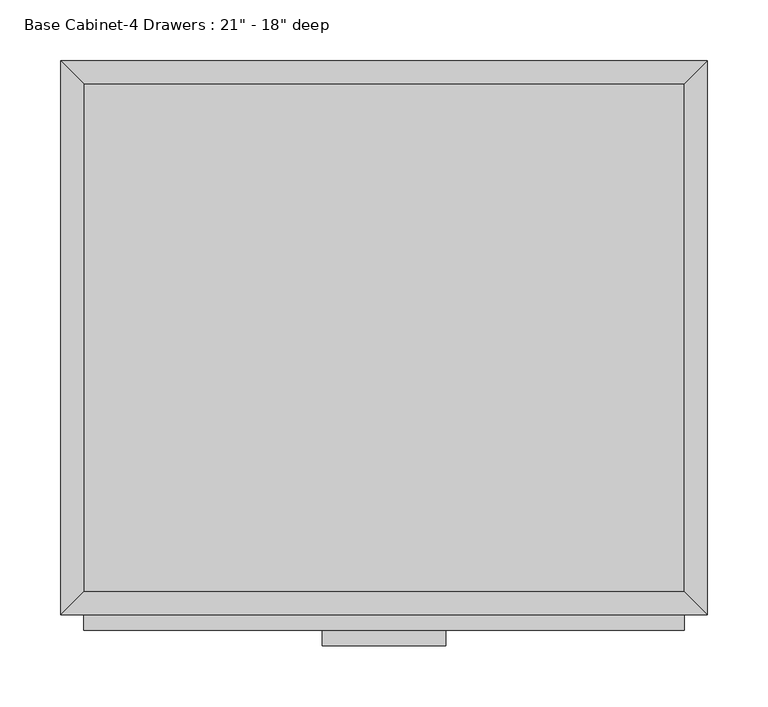
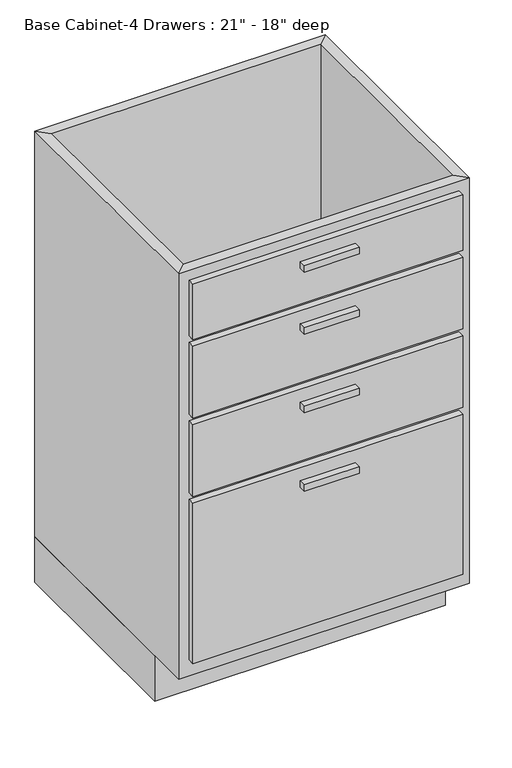
"""IFC4 building model written with IfcOpenShell, lengths in millimetres: furniture geometry."""

from ifc_helpers import new_model, si_unit, frame, origin, origin_with_axes, place, context, project, spatial, polyline, outline, extrude, faceted_brep, source, transform, mapped, element, save


def furniture_18bf1685(model_context):
    return source(origin(), model_context, "Body", "SolidModel", [
        extrude(outline(polyline([(69.5377049, -482.6), (-32.0622951, -482.6), (-32.0622951, -469.9), (69.5377049, -469.9), (69.5377049, -482.6)])), frame((0.0, 0.0, 819.15), z_axis=(0.0, 0.0, 1.0), x_axis=(1.0, 0.0, 0.0)), (0.0, 0.0, 1.0), 12.7),
        extrude(outline(polyline([(69.5377049, -482.6), (-32.0622951, -482.6), (-32.0622951, -469.9), (69.5377049, -469.9), (69.5377049, -482.6)])), frame((0.0, 0.0, 698.5), z_axis=(0.0, 0.0, 1.0), x_axis=(1.0, 0.0, 0.0)), (0.0, 0.0, 1.0), 12.7),
        extrude(outline(polyline([(69.5377049, -482.6), (-32.0622951, -482.6), (-32.0622951, -469.9), (69.5377049, -469.9), (69.5377049, -482.6)])), frame((0.0, 0.0, 546.1), z_axis=(0.0, 0.0, 1.0), x_axis=(1.0, 0.0, 0.0)), (0.0, 0.0, 1.0), 12.7),
        extrude(outline(polyline([(69.5377049, -482.6), (-32.0622951, -482.6), (-32.0622951, -469.9), (69.5377049, -469.9), (69.5377049, -482.6)])), frame((0.0, 0.0, 393.7), z_axis=(0.0, 0.0, 1.0), x_axis=(1.0, 0.0, 0.0)), (0.0, 0.0, 1.0), 12.7),
        extrude(outline(polyline([(266.3877049, -469.9), (-228.9122951, -469.9), (-228.9122951, -457.2), (266.3877049, -457.2), (266.3877049, -469.9)])), frame((0.0, 0.0, 749.3), z_axis=(0.0, 0.0, 1.0), x_axis=(1.0, 0.0, 0.0)), (0.0, 0.0, 1.0), 107.95),
        extrude(outline(polyline([(266.3877049, -469.9), (-228.9122951, -469.9), (-228.9122951, -457.2), (266.3877049, -457.2), (266.3877049, -469.9)])), frame((0.0, 0.0, 596.9), z_axis=(0.0, 0.0, 1.0), x_axis=(1.0, 0.0, 0.0)), (0.0, 0.0, 1.0), 139.7),
        extrude(outline(polyline([(266.3877049, -469.9), (-228.9122951, -469.9), (-228.9122951, -457.2), (266.3877049, -457.2), (266.3877049, -469.9)])), frame((0.0, 0.0, 444.5), z_axis=(0.0, 0.0, 1.0), x_axis=(1.0, 0.0, 0.0)), (0.0, 0.0, 1.0), 139.7),
        extrude(outline(polyline([(266.3877049, -469.9), (-228.9122951, -469.9), (-228.9122951, -457.2), (266.3877049, -457.2), (266.3877049, -469.9)])), frame((0.0, 0.0, 120.65), z_axis=(0.0, 0.0, 1.0), x_axis=(1.0, 0.0, 0.0)), (0.0, 0.0, 1.0), 311.15),
        extrude(outline(polyline([(266.3877049, -19.05), (266.3877049, -438.15), (-228.9122951, -438.15), (-228.9122951, -19.05), (266.3877049, -19.05)])), frame((0.0, 0.0, 88.9), z_axis=(0.0, 0.0, 1.0), x_axis=(1.0, 0.0, 0.0)), (0.0, 0.0, 1.0), 19.05),
        faceted_brep([(266.3877049, -438.15, 876.3), (266.3877049, -438.15, 88.9), (-228.9122951, -438.15, 88.9), (-228.9122951, -438.15, 876.3), (285.4377049, -457.2, 876.3), (-247.9622951, -457.2, 876.3), (285.4377049, -457.2, 88.9), (-247.9622951, -457.2, 88.9), (-228.9122951, -19.05, 88.9), (-228.9122951, -19.05, 876.3), (-247.9622951, 0.0, 876.3), (-247.9622951, 0.0, 88.9), (266.3877049, -19.05, 88.9), (266.3877049, -19.05, 876.3), (285.4377049, 0.0, 876.3), (285.4377049, 0.0, 88.9)], [[[0, 1, 2, 3]], [[4, 0, 3, 5]], [[6, 4, 5, 7]], [[1, 6, 7, 2]], [[3, 2, 8, 9]], [[5, 3, 9, 10]], [[7, 5, 10, 11]], [[2, 7, 11, 8]], [[9, 8, 12, 13]], [[10, 9, 13, 14]], [[11, 10, 14, 15]], [[8, 11, 15, 12]], [[13, 12, 1, 0]], [[14, 13, 0, 4]], [[15, 14, 4, 6]], [[12, 15, 6, 1]]]),
        extrude(outline(polyline([(285.4377049, 0.0), (285.4377049, -381.0), (-247.9622951, -381.0), (-247.9622951, 0.0), (285.4377049, 0.0)])), origin_with_axes(), (0.0, 0.0, 1.0), 88.9),
    ])


if __name__ == "__main__":
    model = new_model("IFC4")
    model_context = context("Model", 3, world=origin())
    ifc_project = project(units=[si_unit("LENGTHUNIT", "METRE", prefix="MILLI")], contexts=[model_context])
    site = spatial("IfcSite", under=ifc_project)
    building = spatial("IfcBuilding", under=site)
    placement = place(None, origin())
    furniture_shape = furniture_18bf1685(model_context)
    element("IfcFurniture", 1, ObjectType="Base Cabinet-4 Drawers : 21\" - 18\" deep", at=placement, inside=building, context=model_context, shape_type="MappedRepresentation", body=[
        mapped(furniture_shape, transform((0.0, 0.0, 0.0), x_axis=(1.0, 0.0, 0.0), y_axis=(0.0, 1.0, 0.0), z_axis=(0.0, 0.0, 1.0))),
    ])
    save(model, "model.ifc")

# Revit data of these elements
# Type "Base Cabinet-4 Drawers : 21\" - 18\" deep"
#   COBie.Type.CreatedBy = "doug.wood@us.ibm.com"
#   COBie.Type.CreatedOn = "2016-04-14T02:07:23"
#   COBie.Type.Name = "Casework_Base Cabinet-4 Drawers_21\" - 18\" deep"
#   COBie.Type.Category = "23-40 35 17 47 11 : Kitchen Casework"
#   COBie.Type.Description = "Base Cabinet-4 Drawers_21\" - 18\" deep"
#   COBie.Type.Manufacturer = ""
#   COBie.Type.ModelNumber = ""
#   Assembly Code = "C1030410"
#   COBie.Type.ReplacementCost = 0
#   Depth = 1' - 6"
#   Height = 2' - 10 1/2"
#   Toe Depth = 0' - 3"
#   Toe Height = 0' - 3 1/2"
#   Width = 1' - 9"
#   COBie.Type = no
#   Cabinet Material = none
#   Door/Drawer Material = none
#   Handle Material = Cabinets - Handles
# Element 1 (IfcFurniture, "Base Cabinet-4 Drawers : 21\" - 18\" deep")
#   Materials on its faces: "Cabinets", "Cabinets - Handles"
# Materials
#   "Cabinets - Handles": class "Metal", colour RGB 57 57 57, transparency 0
#   "Cabinets": class "Miscellaneous", colour RGB 249 249 249, transparency 0
